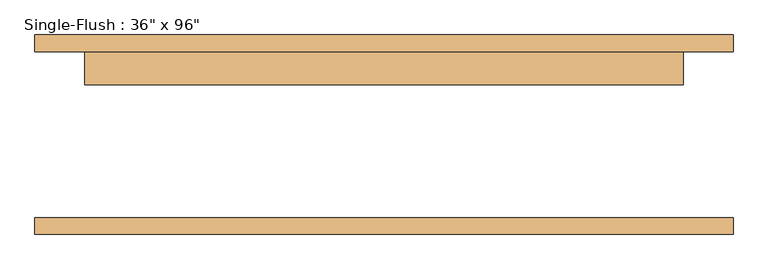
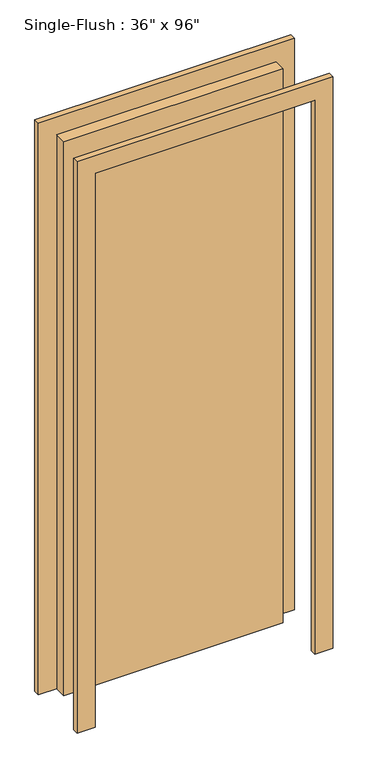
"""IFC4 building model written with IfcOpenShell, lengths in millimetres: door geometry."""

from ifc_helpers import new_model, si_unit, frame, origin, origin_with_axes, place, context, project, spatial, polyline, outline, extrude, source, transform, mapped, element, save


def door_9b482831(model_context):
    return source(origin(), model_context, "Body", "SweptSolid", [
        extrude(outline(polyline([(2514.6, -533.4), (0.0, -533.4), (0.0, -457.2), (2438.4, -457.2), (2438.4, 457.2), (0.0, 457.2), (0.0, 533.4), (2514.6, 533.4), (2514.6, -533.4)])), frame((0.0, 127.0, 0.0), z_axis=(0.0, 1.0, 0.0), x_axis=(0.0, 0.0, 1.0)), (0.0, 0.0, 1.0), 25.4),
        extrude(outline(polyline([(2514.6, 533.4), (2514.6, -533.4), (0.0, -533.4), (0.0, -457.2), (2438.4, -457.2), (2438.4, 457.2), (0.0, 457.2), (0.0, 533.4), (2514.6, 533.4)])), frame((0.0, -152.4, 0.0), z_axis=(0.0, 1.0, 0.0), x_axis=(0.0, 0.0, 1.0)), (0.0, 0.0, 1.0), 25.4),
        extrude(outline(polyline([(457.2, 76.2), (-457.2, 76.2), (-457.2, 127.0), (457.2, 127.0), (457.2, 76.2)])), origin_with_axes(), (0.0, 0.0, 1.0), 2438.4),
    ])


if __name__ == "__main__":
    model = new_model("IFC4")
    model_context = context("Model", 3, world=origin())
    ifc_project = project(units=[si_unit("LENGTHUNIT", "METRE", prefix="MILLI")], contexts=[model_context])
    site = spatial("IfcSite", under=ifc_project)
    building = spatial("IfcBuilding", under=site)
    placement = place(None, origin())
    door_shape = door_9b482831(model_context)
    element("IfcDoor", 1, ObjectType="Single-Flush : 36\" x 96\"", at=placement, inside=building, context=model_context, shape_type="MappedRepresentation", body=[
        mapped(door_shape, transform((0.0, 0.0, 0.0), x_axis=(1.0, 0.0, 0.0), y_axis=(0.0, 1.0, 0.0), z_axis=(0.0, 0.0, 1.0))),
    ])
    save(model, "model.ifc")

# Revit data of these elements
# Type "Single-Flush : 36\" x 96\""
#   Type Mark = "40"
#   Assembly Code = "C1020"
#   Thickness = 50.8 mm
#   Height = 2438.4 mm
#   Trim Projection Ext = 25.4 mm
#   Trim Projection Int = 25.4 mm
#   Trim Width = 76.2 mm
#   Width = 914.4 mm
#   Door Material = Door - Panel
#   Frame Material = Door - Frame
#   Function = (empty or 0)
#   Wall Closure = (empty or 0)
# Element 1 (IfcDoor, "Single-Flush : 36\" x 96\"")
#   Materials on its faces: "Door - Frame", "Door - Panel"
# Materials
#   "Door - Panel": class "Wood", colour RGB 210 159 95, transparency 0
#   "Door - Frame": class "Miscellaneous", colour RGB 118 70 51, transparency 0
